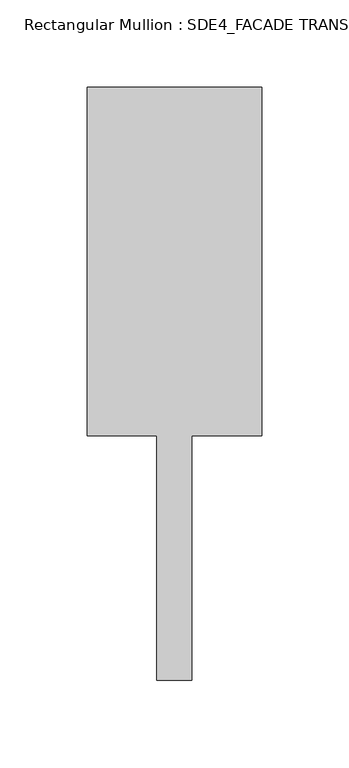
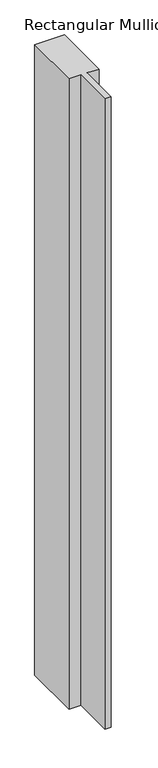
"""IFC4 building model written with IfcOpenShell, lengths in millimetres: member geometry, Rectangular Mullion : SDE4_FACADE TRANSOM TYPE 1."""

from ifc_helpers import new_model, si_unit, frame, origin, place, context, project, spatial, polyline, outline, extrude, source, transform, mapped, element, save


def rectangular_mullion_sde4_facade_transom_type_1_8e8385db(model_context):
    return source(origin(), model_context, "Body", "SweptSolid", [
        extrude(outline(polyline([(50.0, 132.5), (50.0, -67.5), (10.0, -67.5), (10.0, -207.5), (-10.0, -207.5), (-10.0, -67.5), (-50.0, -67.5), (-50.0, 132.5), (50.0, 132.5)])), frame((0.0, 0.0, -2239.0), z_axis=(0.0, 0.0, 1.0), x_axis=(1.0, 0.0, 0.0)), (0.0, 0.0, 1.0), 2239.0),
    ])


if __name__ == "__main__":
    model = new_model("IFC4")
    model_context = context("Model", 3, world=origin())
    ifc_project = project(units=[si_unit("LENGTHUNIT", "METRE", prefix="MILLI")], contexts=[model_context])
    site = spatial("IfcSite", under=ifc_project)
    building = spatial("IfcBuilding", under=site)
    placement = place(None, origin())
    rectangular_mullion_sde4_facade_transom_type_1_shape = rectangular_mullion_sde4_facade_transom_type_1_8e8385db(model_context)
    element("IfcMember", 1, ObjectType="Rectangular Mullion : SDE4_FACADE TRANSOM TYPE 1", at=placement, inside=building, context=model_context, shape_type="MappedRepresentation", body=[
        mapped(rectangular_mullion_sde4_facade_transom_type_1_shape, transform((0.0, 0.0, 0.0), x_axis=(1.0, 0.0, 0.0), y_axis=(0.0, 1.0, 0.0), z_axis=(0.0, 0.0, 1.0))),
    ])
    save(model, "model.ifc")

# Revit data of these elements
# Type "Rectangular Mullion : SDE4_FACADE TRANSOM TYPE 1"
#   built-in parameter 1007322 = 1.11549 (stored number, unit not read)
#   built-in parameter 1007321 = 0.164042 (stored number, unit not read)
#   built-in parameter 1007320 = 0.164042 (stored number, unit not read)
